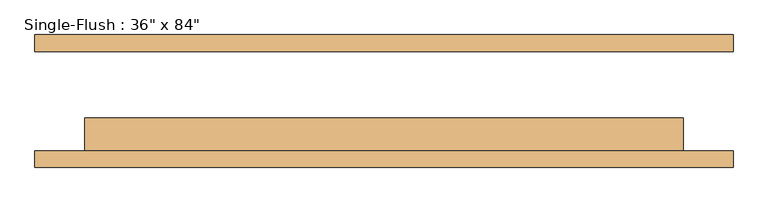
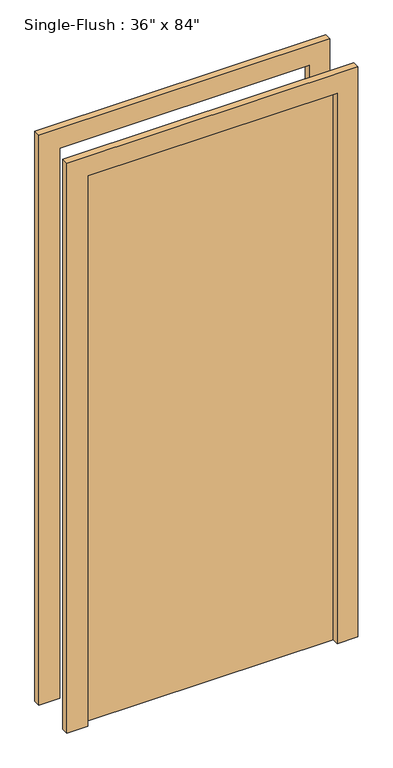
"""IFC4 building model written with IfcOpenShell, lengths in millimetres: door geometry."""

import ifcopenshell
import ifcopenshell.guid

model = None  # the IFC model being written
_history = None  # IfcOwnerHistory: only IFC2X3 demands one
_inside = {}  # id of a spatial element -> (the spatial element, [elements in it])
_under = {}  # id of a project, library or spatial element -> (it, [spatial elements below it])
_declared = {}  # id of a project -> (the project, [libraries it declares])
_typed = {}  # id of a type object -> (the type object, [elements of that type])
_made_of = {}  # id of a material, layer set ... -> (it, [elements and type objects made of it])


def new_model(schema):
    """Start an empty IFC model of exactly this schema.

    Asked for "IFC4X3", IfcOpenShell would pick the latest addendum, in which some entities
    have other attributes; the version numbers below select the first issue.
    IFC2X3 requires an IfcOwnerHistory on every rooted entity: one is made here for all.
    """
    global model, _history
    if schema == "IFC4X3":
        model = ifcopenshell.file(schema_version=(4, 3, 0, 0))
    else:
        model = ifcopenshell.file(schema=schema)
    _inside.clear()
    _under.clear()
    _declared.clear()
    _typed.clear()
    _made_of.clear()
    _history = None
    if model.schema == "IFC2X3":
        org = make("IfcOrganization", Name="unknown")
        user = make(
            "IfcPersonAndOrganization",
            ThePerson=make("IfcPerson", FamilyName="unknown"),
            TheOrganization=org,
        )
        app = make(
            "IfcApplication",
            ApplicationDeveloper=org,
            Version="unknown",
            ApplicationFullName="unknown",
            ApplicationIdentifier="unknown",
        )
        _history = make(
            "IfcOwnerHistory",
            OwningUser=user,
            OwningApplication=app,
            ChangeAction="ADDED",
            CreationDate=0,
        )
    return model


def make(cls, **values):
    """One entity of the class cls with the attributes given. An attribute that is None is left unset."""
    return model.create_entity(
        cls, **{name: value for name, value in values.items() if value is not None}
    )


def rooted(cls, **values):
    """An entity with a GlobalId (a new one), such as an element, a storey or a relation."""
    return make(cls, GlobalId=ifcopenshell.guid.new(), OwnerHistory=_history, **values)


def si_unit(unit_type, name, prefix=None):
    """IfcSIUnit, for example si_unit("LENGTHUNIT", "METRE", prefix="MILLI")."""
    return make("IfcSIUnit", UnitType=unit_type, Prefix=prefix, Name=name)


def assignment(units):
    """IfcUnitAssignment: the units of a project."""
    return None if units is None else make("IfcUnitAssignment", Units=units)


def point(xyz):
    """IfcCartesianPoint."""
    return None if xyz is None else make("IfcCartesianPoint", Coordinates=xyz)


def direction(xyz):
    """IfcDirection."""
    return None if xyz is None else make("IfcDirection", DirectionRatios=xyz)


def frame(location, z_axis=None, x_axis=None):
    """IfcAxis2Placement3D, a coordinate frame: its origin and axes. An axis left out is left unset."""
    return make(
        "IfcAxis2Placement3D",
        Location=point(location),
        Axis=direction(z_axis),
        RefDirection=direction(x_axis),
    )


def origin():
    """The frame at (0, 0, 0) with its axes left unset."""
    return frame((0.0, 0.0, 0.0))


def origin_with_axes():
    """The frame at (0, 0, 0) with the z axis (0, 0, 1) and the x axis (1, 0, 0) written out."""
    return frame((0.0, 0.0, 0.0), z_axis=(0.0, 0.0, 1.0), x_axis=(1.0, 0.0, 0.0))


def place(relative_to, where):
    """IfcLocalPlacement: puts the frame where relative to a parent placement (None: the world)."""
    return make(
        "IfcLocalPlacement", PlacementRelTo=relative_to, RelativePlacement=where
    )


def context(
    kind, dimensions, precision=None, world=None, true_north=None, identifier=None
):
    """IfcGeometricRepresentationContext, for example the 3D "Model" context."""
    return make(
        "IfcGeometricRepresentationContext",
        ContextIdentifier=identifier,
        ContextType=kind,
        CoordinateSpaceDimension=dimensions,
        Precision=precision,
        WorldCoordinateSystem=world,
        TrueNorth=true_north,
    )


def project(units=None, contexts=None):
    """IfcProject with its units and contexts."""
    return rooted(
        "IfcProject",
        Name="project",
        RepresentationContexts=contexts,
        UnitsInContext=assignment(units),
    )


def spatial(cls, under=None, at=None, **own):
    """A site, building, storey or space (cls), placed at a placement, below another one or the project."""
    s = rooted(cls, ObjectPlacement=at, **own)
    if under is not None:
        _under.setdefault(under.id(), (under, []))[1].append(s)
    return s


def polyline(points):
    """IfcPolyline through the points."""
    return make("IfcPolyline", Points=[point(p) for p in points])


def outline(outer, holes=None, kind="AREA"):
    """IfcArbitraryClosedProfileDef: a profile drawn as a closed curve; with holes, ...WithVoids."""
    if holes is None:
        return make("IfcArbitraryClosedProfileDef", ProfileType=kind, OuterCurve=outer)
    return make(
        "IfcArbitraryProfileDefWithVoids",
        ProfileType=kind,
        OuterCurve=outer,
        InnerCurves=holes,
    )


def extrude(swept, where, along, depth):
    """IfcExtrudedAreaSolid: the profile swept, set in the frame where, extruded along a direction by depth."""
    return make(
        "IfcExtrudedAreaSolid",
        SweptArea=swept,
        Position=where,
        ExtrudedDirection=direction(along),
        Depth=depth,
    )


def shape(context_of_items, identifier, shape_type, items):
    """IfcShapeRepresentation: the items that make up one representation, for example the "Body"."""
    return make(
        "IfcShapeRepresentation",
        ContextOfItems=context_of_items,
        RepresentationIdentifier=identifier,
        RepresentationType=shape_type,
        Items=items,
    )


def source(mapping_origin, context_of_items, identifier, shape_type, items):
    """IfcRepresentationMap: a shape defined once, which mapped items show again and again."""
    return make(
        "IfcRepresentationMap",
        MappingOrigin=mapping_origin,
        MappedRepresentation=shape(context_of_items, identifier, shape_type, items),
    )


def transform(
    local_origin,
    x_axis=None,
    y_axis=None,
    z_axis=None,
    scale=None,
    scale2=None,
    scale3=None,
    uniform=True,
):
    """IfcCartesianTransformationOperator3D, or its non-uniform kind. x_axis, y_axis, z_axis: its Axis1, 2, 3."""
    if uniform:
        return make(
            "IfcCartesianTransformationOperator3D",
            Axis1=direction(x_axis),
            Axis2=direction(y_axis),
            LocalOrigin=point(local_origin),
            Scale=scale,
            Axis3=direction(z_axis),
        )
    return make(
        "IfcCartesianTransformationOperator3DnonUniform",
        Axis1=direction(x_axis),
        Axis2=direction(y_axis),
        LocalOrigin=point(local_origin),
        Scale=scale,
        Axis3=direction(z_axis),
        Scale2=scale2,
        Scale3=scale3,
    )


def mapped(mapping_source, mapping_target):
    """IfcMappedItem: shows the shape of a source again, moved by a transform."""
    return make(
        "IfcMappedItem", MappingSource=mapping_source, MappingTarget=mapping_target
    )


def made_of(thing, what):
    """Note that an element or type object is made of a material, layer set ...; save() writes the relation."""
    if what is not None:
        _made_of.setdefault(what.id(), (what, []))[1].append(thing)
    return thing


def element(
    cls,
    number,
    at=None,
    inside=None,
    cuts=None,
    type_object=None,
    material=None,
    context=None,
    identifier="Body",
    shape_type=None,
    held_by="IfcProductDefinitionShape",
    body=None,
    shapes=None,
    **own,
):
    """One element of the class cls, such as IfcWall. Its Tag is "e" and its number.

    at: its placement. inside: the storey or other place that contains it. cuts: it is an
    opening in that element (IfcRelVoidsElement). A single representation is given by context,
    identifier, shape_type and body (its items); several are given by shapes. held_by: the class
    of the entity that holds the representations. save() writes the other relations.
    """
    e = rooted(cls, Tag="e%d" % number, ObjectPlacement=at, **own)
    if body is not None:
        shapes = [shape(context, identifier, shape_type, body)]
    if shapes is not None:
        e.Representation = make(held_by, Representations=shapes)
    if inside is not None:
        _inside.setdefault(inside.id(), (inside, []))[1].append(e)
    if cuts is not None:
        rooted(
            "IfcRelVoidsElement", RelatingBuildingElement=cuts, RelatedOpeningElement=e
        )
    if type_object is not None:
        _typed.setdefault(type_object.id(), (type_object, []))[1].append(e)
    return made_of(e, material)


def aggregate(whole, parts):
    """IfcRelAggregates: a whole, such as a stair, and the parts it consists of."""
    return rooted("IfcRelAggregates", RelatingObject=whole, RelatedObjects=parts)


def save(model, path):
    """Write the relations noted so far, then the file.

    IfcRelAggregates (storeys below a building ...), IfcRelContainedInSpatialStructure (elements
    in a storey), IfcRelDefinesByType, IfcRelAssociatesMaterial and IfcRelDeclares: one each for
    every whole, place, type object, material and project.
    """
    for whole, parts in _under.values():
        aggregate(whole, parts)
    for where, things in _inside.values():
        rooted(
            "IfcRelContainedInSpatialStructure",
            RelatedElements=things,
            RelatingStructure=where,
        )
    for kind, things in _typed.values():
        rooted("IfcRelDefinesByType", RelatedObjects=things, RelatingType=kind)
    for what, things in _made_of.values():
        rooted("IfcRelAssociatesMaterial", RelatedObjects=things, RelatingMaterial=what)
    for by, libraries in _declared.values():
        rooted("IfcRelDeclares", RelatingContext=by, RelatedDefinitions=libraries)
    model.write(path)


def door_686f89d2(model_context):
    return source(origin(), model_context, "Body", "SweptSolid", [
        extrude(outline(polyline([(2209.8, -533.4), (0.0, -533.4), (0.0, -457.2), (2133.6, -457.2), (2133.6, 457.2), (0.0, 457.2), (0.0, 533.4), (2209.8, 533.4), (2209.8, -533.4)])), frame((0.0, -101.6, 0.0), z_axis=(0.0, 1.0, 0.0), x_axis=(0.0, 0.0, 1.0)), (0.0, 0.0, 1.0), 25.4),
        extrude(outline(polyline([(2209.8, 533.4), (2209.8, -533.4), (0.0, -533.4), (0.0, -457.2), (2133.6, -457.2), (2133.6, 457.2), (0.0, 457.2), (0.0, 533.4), (2209.8, 533.4)])), frame((0.0, 76.2, 0.0), z_axis=(0.0, 1.0, 0.0), x_axis=(0.0, 0.0, 1.0)), (0.0, 0.0, 1.0), 25.4),
        extrude(outline(polyline([(457.2, -25.4), (457.2, -76.2), (-457.2, -76.2), (-457.2, -25.4), (457.2, -25.4)])), origin_with_axes(), (0.0, 0.0, 1.0), 2133.6),
    ])


if __name__ == "__main__":
    model = new_model("IFC4")
    model_context = context("Model", 3, world=origin())
    ifc_project = project(units=[si_unit("LENGTHUNIT", "METRE", prefix="MILLI")], contexts=[model_context])
    site = spatial("IfcSite", under=ifc_project)
    building = spatial("IfcBuilding", under=site)
    placement = place(None, origin())
    door_shape = door_686f89d2(model_context)
    element("IfcDoor", 1, ObjectType="Single-Flush : 36\" x 84\"", at=placement, inside=building, context=model_context, shape_type="MappedRepresentation", body=[
        mapped(door_shape, transform((0.0, 0.0, 0.0), x_axis=(1.0, 0.0, 0.0), y_axis=(0.0, 1.0, 0.0), z_axis=(0.0, 0.0, 1.0))),
    ])
    save(model, "model.ifc")

# Revit data of these elements
# Type "Single-Flush : 36\" x 84\""
#   Type Mark = "1"
#   Assembly Code = "C1020"
#   Thickness = 50.8 mm
#   Height = 2133.6 mm
#   Trim Projection Ext = 25.4 mm
#   Trim Projection Int = 25.4 mm
#   Trim Width = 76.2 mm
#   Width = 914.4 mm
#   Door Material = Door - Panel
#   Frame Material = Door - Frame
#   Function = (empty or 0)
#   Wall Closure = (empty or 0)
# Element 1 (IfcDoor, "Single-Flush : 36\" x 84\"")
#   Materials on its faces: "Door - Frame", "Door - Panel"
# Materials
#   "Door - Panel": class "Wood", colour RGB 210 159 95, transparency 0
#   "Door - Frame": class "Miscellaneous", colour RGB 118 70 51, transparency 0
